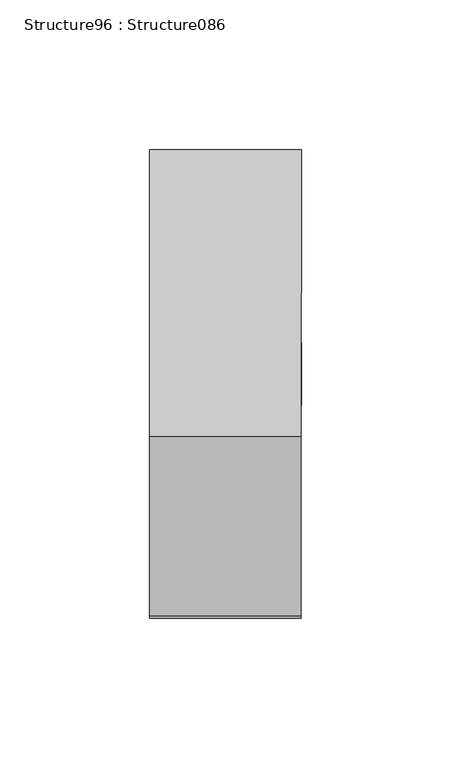
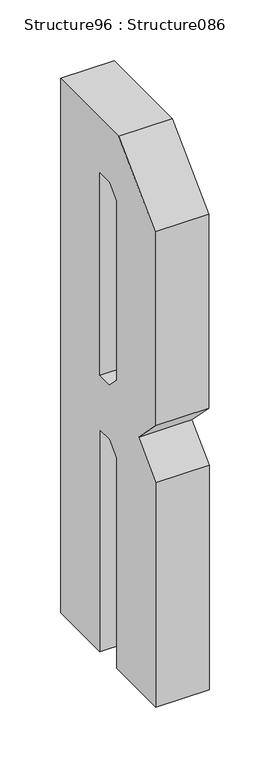
"""IFC4 building model written with IfcOpenShell, lengths in millimetres: proxy geometry, Structure96 : Structure086."""

from ifc_helpers import new_model, si_unit, frame, origin, place, context, project, spatial, polyline, outline, extrude, source, transform, mapped, element, save


def structure96_structure086_58963b22(model_context):
    return source(origin(), model_context, "Body", "SweptSolid", [
        extrude(outline(polyline([(225.8643819, 0.0), (225.8643819, -64.5407118), (13.8227312, -64.5407118), (2.2982141, -76.0652289), (2.2982141, -92.2007628), (225.8643819, -92.2007628), (225.8643819, -156.7268861), (-311.916648, -156.7268861), (-311.916648, -60.6961224), (-251.9962041, -0.7756784), (-56.8607841, -0.7756784), (-28.4303921, -28.4303921), (0.0, 0.0), (225.8643819, 0.0)]), holes=[polyline([(-52.2437186, -92.2007628), (-52.2437186, -76.8327236), (-63.769659, -65.3067832), (-244.3166322, -65.3067832), (-255.8411493, -76.8313003), (-255.8411493, -92.2007628), (-52.2437186, -92.2007628)])]), frame((-56110.0449044, 290829.8503882, 59.1178087), z_axis=(-0.9999998917542984, 0.00046528635450596156, 0.0), x_axis=(0.0, 0.0, -1.0)), (0.0, 0.0, 1.0), 50.8),
    ])


if __name__ == "__main__":
    model = new_model("IFC4")
    model_context = context("Model", 3, world=origin())
    ifc_project = project(units=[si_unit("LENGTHUNIT", "METRE", prefix="MILLI")], contexts=[model_context])
    site = spatial("IfcSite", under=ifc_project)
    building = spatial("IfcBuilding", under=site)
    placement = place(None, origin())
    structure96_structure086_shape = structure96_structure086_58963b22(model_context)
    element("IfcBuildingElementProxy", 1, Name="Structure96 : Structure086", ObjectType="Structure96 : Structure086", at=placement, inside=building, context=model_context, shape_type="MappedRepresentation", body=[
        mapped(structure96_structure086_shape, transform((0.0, 0.0, 0.0), x_axis=(1.0, 0.0, 0.0), y_axis=(0.0, 1.0, 0.0), z_axis=(0.0, 0.0, 1.0))),
    ])
    save(model, "model.ifc")

# Revit data of these elements
# Type "Structure96 : Structure086"
#   NameOverride = "Structure086"
# Element 1 (IfcBuildingElementProxy, "Structure96 : Structure086")
#   Materials on its faces: "BRUSHED ALUMINUM LETTERING"
# Materials
#   "BRUSHED ALUMINUM LETTERING": class "Unassigned", colour RGB 169 181 186, transparency 0, Cost = 0
